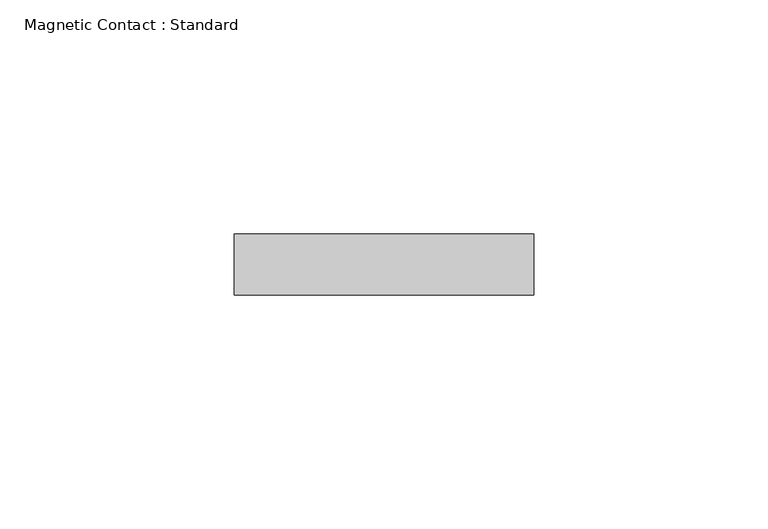
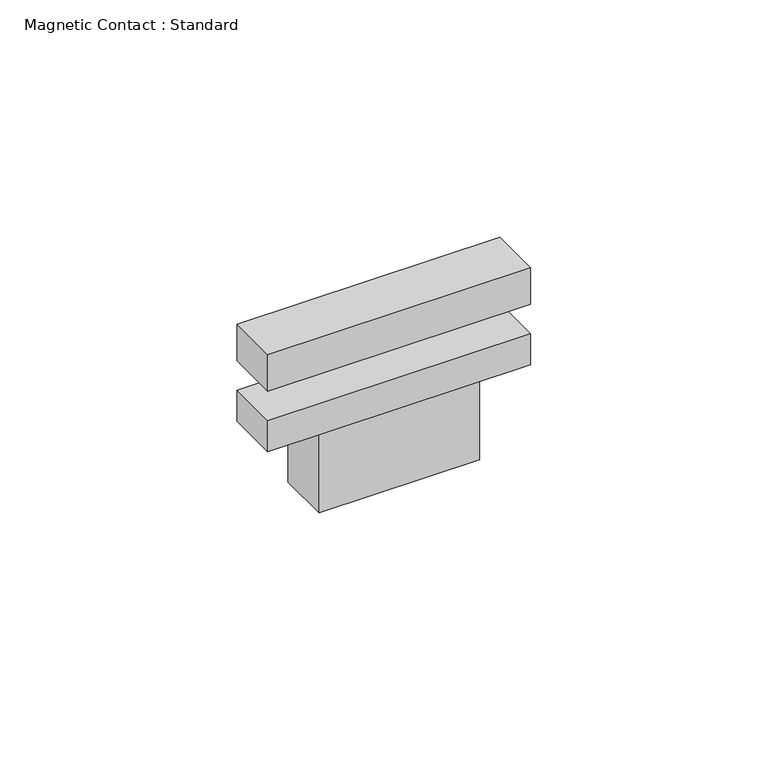
"""IFC4 building model written with IfcOpenShell, lengths in millimetres: proxy geometry, Magnetic Contact : Standard."""

from ifc_helpers import new_model, si_unit, frame, origin, origin_with_axes, place, context, project, spatial, polyline, outline, extrude, source, transform, mapped, element, save


def magnetic_contact_standard_5e95dac8(model_context):
    return source(origin(), model_context, "Body", "SweptSolid", [
        extrude(outline(polyline([(32.0, -13.0), (-32.0, -13.0), (-32.0, 0.0), (32.0, 0.0), (32.0, -13.0)])), frame((0.0, 0.0, 15.5767529), z_axis=(0.0, 0.0, 1.0), x_axis=(1.0, 0.0, 0.0)), (0.0, 0.0, 1.0), 9.4232471),
        extrude(outline(polyline([(32.0, -13.0), (-32.0, -13.0), (-32.0, 0.0), (32.0, 0.0), (32.0, -13.0)])), origin_with_axes(), (0.0, 0.0, 1.0), 8.0),
        extrude(outline(polyline([(19.5, -13.0), (-19.5, -13.0), (-19.5, 0.0), (19.5, 0.0), (19.5, -13.0)])), frame((0.0, 0.0, -20.0), z_axis=(0.0, 0.0, 1.0), x_axis=(1.0, 0.0, 0.0)), (0.0, 0.0, 1.0), 20.0),
    ])


if __name__ == "__main__":
    model = new_model("IFC4")
    model_context = context("Model", 3, world=origin())
    ifc_project = project(units=[si_unit("LENGTHUNIT", "METRE", prefix="MILLI")], contexts=[model_context])
    site = spatial("IfcSite", under=ifc_project)
    building = spatial("IfcBuilding", under=site)
    placement = place(None, origin())
    magnetic_contact_standard_shape = magnetic_contact_standard_5e95dac8(model_context)
    element("IfcBuildingElementProxy", 1, Name="Magnetic Contact : Standard", ObjectType="Magnetic Contact : Standard", at=placement, inside=building, context=model_context, shape_type="MappedRepresentation", body=[
        mapped(magnetic_contact_standard_shape, transform((0.0, 0.0, 0.0), x_axis=(1.0, 0.0, 0.0), y_axis=(0.0, 1.0, 0.0), z_axis=(0.0, 0.0, 1.0))),
    ])
    save(model, "model.ifc")

# Revit data of these elements
# Type "Magnetic Contact : Standard"
#   Type Mark = "Magnetic Contact"
#   Classification.OmniClass.23.Number = "23-29 11 21"
#   Classification.OmniClass.23.Description = "Security Sensors"
#   COBie.Type.CreatedBy = "info@mma.ie"
#   COBie.Type.CreatedOn = "2017-07-26T09:12:44"
#   COBie.Type.Name = "Magnetic Contact"
#   COBie.Type.Category = "23-29 11 21 : Security Sensors"
#   COBie.Type.Description = "Magnetic Contact_Standard"
#   COBie.Type.AssetType = "Fixed"
#   COBie.Type.Manufacturer = ""
#   COBie.Type.ModelNumber = ""
#   Keynote = "41 24 33.A"
#   COBie.Type.ReplacementCost = 0
#   MC_Width = 64 mm
#   MC_Height = 25 mm
#   MC_Depth = 13 mm
#   Default Elevation = 1200 mm
#   COBie.Type = yes
#   URL = ""
#   Model = ""
#   Manufacturer = ""
